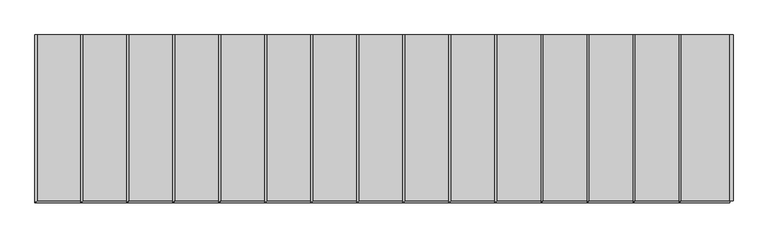
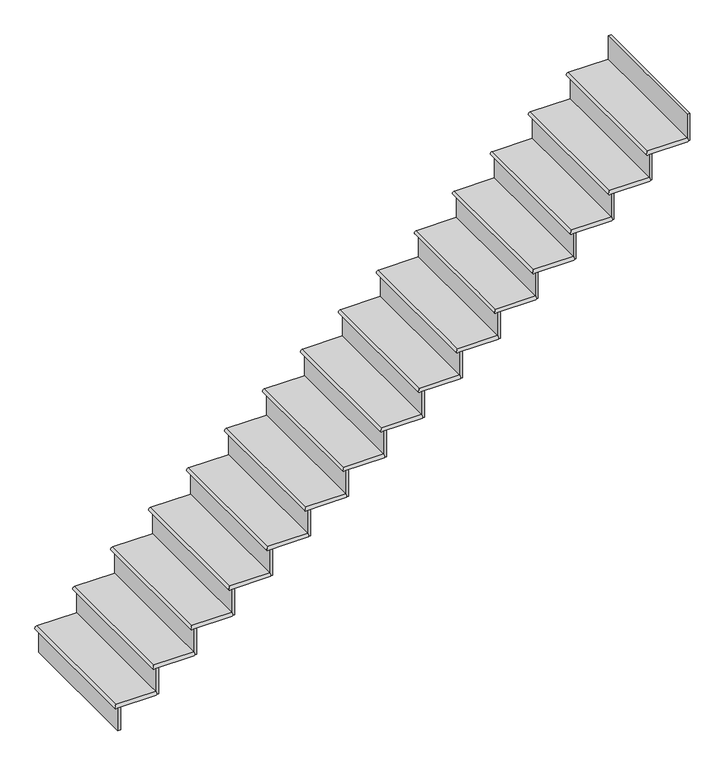
"""IFC4 building model written with IfcOpenShell, lengths in millimetres: stair flight geometry."""

import ifcopenshell
import ifcopenshell.guid

model = None  # the IFC model being written
_history = None  # IfcOwnerHistory: only IFC2X3 demands one
_inside = {}  # id of a spatial element -> (the spatial element, [elements in it])
_under = {}  # id of a project, library or spatial element -> (it, [spatial elements below it])
_declared = {}  # id of a project -> (the project, [libraries it declares])
_typed = {}  # id of a type object -> (the type object, [elements of that type])
_made_of = {}  # id of a material, layer set ... -> (it, [elements and type objects made of it])


def new_model(schema):
    """Start an empty IFC model of exactly this schema.

    Asked for "IFC4X3", IfcOpenShell would pick the latest addendum, in which some entities
    have other attributes; the version numbers below select the first issue.
    IFC2X3 requires an IfcOwnerHistory on every rooted entity: one is made here for all.
    """
    global model, _history
    if schema == "IFC4X3":
        model = ifcopenshell.file(schema_version=(4, 3, 0, 0))
    else:
        model = ifcopenshell.file(schema=schema)
    _inside.clear()
    _under.clear()
    _declared.clear()
    _typed.clear()
    _made_of.clear()
    _history = None
    if model.schema == "IFC2X3":
        org = make("IfcOrganization", Name="unknown")
        user = make(
            "IfcPersonAndOrganization",
            ThePerson=make("IfcPerson", FamilyName="unknown"),
            TheOrganization=org,
        )
        app = make(
            "IfcApplication",
            ApplicationDeveloper=org,
            Version="unknown",
            ApplicationFullName="unknown",
            ApplicationIdentifier="unknown",
        )
        _history = make(
            "IfcOwnerHistory",
            OwningUser=user,
            OwningApplication=app,
            ChangeAction="ADDED",
            CreationDate=0,
        )
    return model


def make(cls, **values):
    """One entity of the class cls with the attributes given. An attribute that is None is left unset."""
    return model.create_entity(
        cls, **{name: value for name, value in values.items() if value is not None}
    )


def rooted(cls, **values):
    """An entity with a GlobalId (a new one), such as an element, a storey or a relation."""
    return make(cls, GlobalId=ifcopenshell.guid.new(), OwnerHistory=_history, **values)


def si_unit(unit_type, name, prefix=None):
    """IfcSIUnit, for example si_unit("LENGTHUNIT", "METRE", prefix="MILLI")."""
    return make("IfcSIUnit", UnitType=unit_type, Prefix=prefix, Name=name)


def assignment(units):
    """IfcUnitAssignment: the units of a project."""
    return None if units is None else make("IfcUnitAssignment", Units=units)


def point(xyz):
    """IfcCartesianPoint."""
    return None if xyz is None else make("IfcCartesianPoint", Coordinates=xyz)


def direction(xyz):
    """IfcDirection."""
    return None if xyz is None else make("IfcDirection", DirectionRatios=xyz)


def frame(location, z_axis=None, x_axis=None):
    """IfcAxis2Placement3D, a coordinate frame: its origin and axes. An axis left out is left unset."""
    return make(
        "IfcAxis2Placement3D",
        Location=point(location),
        Axis=direction(z_axis),
        RefDirection=direction(x_axis),
    )


def origin():
    """The frame at (0, 0, 0) with its axes left unset."""
    return frame((0.0, 0.0, 0.0))


def place(relative_to, where):
    """IfcLocalPlacement: puts the frame where relative to a parent placement (None: the world)."""
    return make(
        "IfcLocalPlacement", PlacementRelTo=relative_to, RelativePlacement=where
    )


def context(
    kind, dimensions, precision=None, world=None, true_north=None, identifier=None
):
    """IfcGeometricRepresentationContext, for example the 3D "Model" context."""
    return make(
        "IfcGeometricRepresentationContext",
        ContextIdentifier=identifier,
        ContextType=kind,
        CoordinateSpaceDimension=dimensions,
        Precision=precision,
        WorldCoordinateSystem=world,
        TrueNorth=true_north,
    )


def project(units=None, contexts=None):
    """IfcProject with its units and contexts."""
    return rooted(
        "IfcProject",
        Name="project",
        RepresentationContexts=contexts,
        UnitsInContext=assignment(units),
    )


def spatial(cls, under=None, at=None, **own):
    """A site, building, storey or space (cls), placed at a placement, below another one or the project."""
    s = rooted(cls, ObjectPlacement=at, **own)
    if under is not None:
        _under.setdefault(under.id(), (under, []))[1].append(s)
    return s


def circle_curve(where, radius):
    """IfcCircle in the frame where."""
    return make("IfcCircle", Position=where, Radius=radius)


def ellipse_curve(where, semi_axis1, semi_axis2):
    """IfcEllipse in the frame where."""
    return make(
        "IfcEllipse", Position=where, SemiAxis1=semi_axis1, SemiAxis2=semi_axis2
    )


def faces_of(points, faces, orient=None, outer=None):
    """IfcFace entities. A face is a list of loops; a loop is a list of indices into points, from 0.

    orient and outer hold one flag for each loop. By default every Orientation is true, the
    first loop of a face is its IfcFaceOuterBound and the others are IfcFaceBound.
    """
    made = []
    for i, loops in enumerate(faces):
        bounds = []
        for j, loop in enumerate(loops):
            is_outer = j == 0 if outer is None else outer[i][j]
            bounds.append(
                make(
                    "IfcFaceOuterBound" if is_outer else "IfcFaceBound",
                    Bound=make("IfcPolyLoop", Polygon=[points[k] for k in loop]),
                    Orientation=True if orient is None else orient[i][j],
                )
            )
        made.append(make("IfcFace", Bounds=bounds))
    return made


def faceted_brep(points, faces, orient=None, outer=None, voids=None):
    """IfcFacetedBrep: a solid bounded by flat faces; with voids (closed shells), ...WithVoids."""
    shared = [point(p) for p in points]
    hull = make("IfcClosedShell", CfsFaces=faces_of(shared, faces, orient, outer))
    if voids is None:
        return make("IfcFacetedBrep", Outer=hull)
    return make(
        "IfcFacetedBrepWithVoids",
        Outer=hull,
        Voids=[
            make(cls, CfsFaces=faces_of(shared, fs, o, b)) for cls, fs, o, b in voids
        ],
    )


def shape(context_of_items, identifier, shape_type, items):
    """IfcShapeRepresentation: the items that make up one representation, for example the "Body"."""
    return make(
        "IfcShapeRepresentation",
        ContextOfItems=context_of_items,
        RepresentationIdentifier=identifier,
        RepresentationType=shape_type,
        Items=items,
    )


def source(mapping_origin, context_of_items, identifier, shape_type, items):
    """IfcRepresentationMap: a shape defined once, which mapped items show again and again."""
    return make(
        "IfcRepresentationMap",
        MappingOrigin=mapping_origin,
        MappedRepresentation=shape(context_of_items, identifier, shape_type, items),
    )


def transform(
    local_origin,
    x_axis=None,
    y_axis=None,
    z_axis=None,
    scale=None,
    scale2=None,
    scale3=None,
    uniform=True,
):
    """IfcCartesianTransformationOperator3D, or its non-uniform kind. x_axis, y_axis, z_axis: its Axis1, 2, 3."""
    if uniform:
        return make(
            "IfcCartesianTransformationOperator3D",
            Axis1=direction(x_axis),
            Axis2=direction(y_axis),
            LocalOrigin=point(local_origin),
            Scale=scale,
            Axis3=direction(z_axis),
        )
    return make(
        "IfcCartesianTransformationOperator3DnonUniform",
        Axis1=direction(x_axis),
        Axis2=direction(y_axis),
        LocalOrigin=point(local_origin),
        Scale=scale,
        Axis3=direction(z_axis),
        Scale2=scale2,
        Scale3=scale3,
    )


def mapped(mapping_source, mapping_target):
    """IfcMappedItem: shows the shape of a source again, moved by a transform."""
    return make(
        "IfcMappedItem", MappingSource=mapping_source, MappingTarget=mapping_target
    )


def made_of(thing, what):
    """Note that an element or type object is made of a material, layer set ...; save() writes the relation."""
    if what is not None:
        _made_of.setdefault(what.id(), (what, []))[1].append(thing)
    return thing


def element(
    cls,
    number,
    at=None,
    inside=None,
    cuts=None,
    type_object=None,
    material=None,
    context=None,
    identifier="Body",
    shape_type=None,
    held_by="IfcProductDefinitionShape",
    body=None,
    shapes=None,
    **own,
):
    """One element of the class cls, such as IfcWall. Its Tag is "e" and its number.

    at: its placement. inside: the storey or other place that contains it. cuts: it is an
    opening in that element (IfcRelVoidsElement). A single representation is given by context,
    identifier, shape_type and body (its items); several are given by shapes. held_by: the class
    of the entity that holds the representations. save() writes the other relations.
    """
    e = rooted(cls, Tag="e%d" % number, ObjectPlacement=at, **own)
    if body is not None:
        shapes = [shape(context, identifier, shape_type, body)]
    if shapes is not None:
        e.Representation = make(held_by, Representations=shapes)
    if inside is not None:
        _inside.setdefault(inside.id(), (inside, []))[1].append(e)
    if cuts is not None:
        rooted(
            "IfcRelVoidsElement", RelatingBuildingElement=cuts, RelatedOpeningElement=e
        )
    if type_object is not None:
        _typed.setdefault(type_object.id(), (type_object, []))[1].append(e)
    return made_of(e, material)


def aggregate(whole, parts):
    """IfcRelAggregates: a whole, such as a stair, and the parts it consists of."""
    return rooted("IfcRelAggregates", RelatingObject=whole, RelatedObjects=parts)


def save(model, path):
    """Write the relations noted so far, then the file.

    IfcRelAggregates (storeys below a building ...), IfcRelContainedInSpatialStructure (elements
    in a storey), IfcRelDefinesByType, IfcRelAssociatesMaterial and IfcRelDeclares: one each for
    every whole, place, type object, material and project.
    """
    for whole, parts in _under.values():
        aggregate(whole, parts)
    for where, things in _inside.values():
        rooted(
            "IfcRelContainedInSpatialStructure",
            RelatedElements=things,
            RelatingStructure=where,
        )
    for kind, things in _typed.values():
        rooted("IfcRelDefinesByType", RelatedObjects=things, RelatingType=kind)
    for what, things in _made_of.values():
        rooted("IfcRelAssociatesMaterial", RelatedObjects=things, RelatingMaterial=what)
    for by, libraries in _declared.values():
        rooted("IfcRelDeclares", RelatingContext=by, RelatedDefinitions=libraries)
    model.write(path)


def plane_surface(at):
    """IfcPlane: the flat surface through the origin of the frame at, square to its z axis."""
    return make("IfcPlane", Position=at)


def cylinder_surface(at, radius):
    """IfcCylindricalSurface: all points at the distance radius from the z axis of the frame at."""
    return make("IfcCylindricalSurface", Position=at, Radius=radius)


def advanced_brep(points, edges, surfaces, faces):
    """IfcAdvancedBrep: a solid bounded by faces that lie on surfaces and meet in shared edges.

    An edge is (start, end): straight between two places in points (the first is 0);
    or (start, end, curve); or (start, end, curve, False) where it runs against its curve.
    A face is (place in surfaces, loops), or (place, loops, False) where it looks against
    its surface's normal. A loop lists edges by number (the first is 1), with a minus sign
    where the edge is run from its end to its start. The first loop is the outer one.
    """
    corners = [point(p) for p in points]
    vertices = [make("IfcVertexPoint", VertexGeometry=c) for c in corners]
    made = []
    for start, end, *more in edges:
        made.append(
            make(
                "IfcEdgeCurve",
                EdgeStart=vertices[start],
                EdgeEnd=vertices[end],
                EdgeGeometry=more[0] if more else make("IfcPolyline", Points=[corners[start], corners[end]]),
                SameSense=more[1] if len(more) > 1 else True,
            )
        )
    hull = []
    for where, loops, *sense in faces:
        bounds = []
        for j, loop in enumerate(loops):
            ring = [make("IfcOrientedEdge", EdgeElement=made[abs(k) - 1], Orientation=k > 0) for k in loop]
            bounds.append(
                make(
                    "IfcFaceOuterBound" if j == 0 else "IfcFaceBound",
                    Bound=make("IfcEdgeLoop", EdgeList=ring),
                    Orientation=True,
                )
            )
        hull.append(make("IfcAdvancedFace", Bounds=bounds, FaceSurface=surfaces[where], SameSense=sense[0] if sense else True))
    return make("IfcAdvancedBrep", Outer=make("IfcClosedShell", CfsFaces=hull))


def stair_flight_f94ab1f9(model_context):
    return source(origin(), model_context, "Body", "SolidModel", [
        advanced_brep(
        [(-27218.1481446, 896.1568972, 165.1), (-27218.1481446, 896.1568972, 190.5), (-27218.1481446, 1810.5568972, 190.5), (-27218.1481446, 1810.5568972, 165.1), (-26951.4481446, 1810.5568972, 190.5), (-26951.4481446, 896.1568972, 190.5), (-26951.4481446, 1810.5568972, 165.1), (-26951.4481446, 896.1568972, 165.1)],
        [
            (0, 1, ellipse_curve(frame((-27218.1481446, 896.1568972, 177.8), z_axis=(-0.7071067811865447, 0.7071067811865502, 0.0), x_axis=(-0.7071067811865501, -0.7071067811865449, 0.0)), 17.9605122, 12.7)),
            (1, 2),
            (2, 3, circle_curve(frame((-27218.1481446, 1810.5568972, 177.8), z_axis=(0.0, -1.0, 0.0), x_axis=(1.0, 0.0, 0.0)), 12.7)),
            (3, 0),
            (4, 2),
            (1, 5),
            (5, 4),
            (3, 6),
            (6, 7),
            (7, 0),
            (4, 6),
            (5, 7, circle_curve(frame((-26951.4481446, 896.1568972, 177.8), z_axis=(1.0, 0.0, 0.0), x_axis=(0.0, 1.0, 0.0)), 12.7)),
        ],
        [
            cylinder_surface(frame((-27218.1481446, 896.1568972, 177.8), z_axis=(0.0, -1.0, 0.0), x_axis=(1.0, 0.0, 0.0)), 12.7),
            plane_surface(frame((-27230.8481446, 1810.5568972, 190.5), z_axis=(0.0, 0.0, 1.0), x_axis=(-1.0, 0.0, 0.0))),
            plane_surface(frame((-27230.8481446, 1810.5568972, 165.1), z_axis=(0.0, 0.0, -1.0), x_axis=(1.0, 0.0, 0.0))),
            plane_surface(frame((-26951.4481446, 1810.5568972, 190.5), z_axis=(0.0, 1.0, 0.0), x_axis=(0.0, 0.0, -1.0))),
            plane_surface(frame((-26951.4481446, 896.1568972, 190.5), z_axis=(1.0, 0.0, 0.0), x_axis=(0.0, 0.0, -1.0))),
            cylinder_surface(frame((-26951.4481446, 896.1568972, 177.8), z_axis=(1.0, 0.0, 0.0), x_axis=(0.0, 1.0, 0.0)), 12.7),
        ],
        [
            (0, [[1, 2, 3, 4]]),
            (1, [[5, -2, 6, 7]]),
            (2, [[8, 9, 10, -4]]),
            (3, [[-5, 11, -8, -3]]),
            (4, [[-7, 12, -9, -11]]),
            (5, [[-12, -6, -1, -10]]),
        ],
    ),
        faceted_brep([(-27205.4481446, 896.1568972, 165.1), (-27205.4481446, 896.1568972, 0.0), (-27186.3981446, 896.1568972, 0.0), (-27186.3981446, 896.1568972, 165.1), (-27205.4481446, 1810.5568972, 165.1), (-27186.3981446, 1810.5568972, 165.1), (-27186.3981446, 1810.5568972, 0.0), (-27205.4481446, 1810.5568972, 0.0)], [[[0, 1, 2, 3]], [[4, 5, 6, 7]], [[1, 0, 4, 7]], [[2, 1, 7, 6]], [[3, 2, 6, 5]], [[0, 3, 5, 4]]]),
        faceted_brep([(-26951.4481446, 896.1568972, 355.6), (-26951.4481446, 896.1568972, 165.1), (-26932.3981446, 896.1568972, 165.1), (-26932.3981446, 896.1568972, 355.6), (-26951.4481446, 1810.5568972, 355.6), (-26932.3981446, 1810.5568972, 355.6), (-26932.3981446, 1810.5568972, 165.1), (-26951.4481446, 1810.5568972, 165.1)], [[[0, 1, 2, 3]], [[4, 5, 6, 7]], [[1, 0, 4, 7]], [[2, 1, 7, 6]], [[3, 2, 6, 5]], [[0, 3, 5, 4]]]),
        advanced_brep(
        [(-26697.4481446, 1810.5568972, 381.0), (-26964.1481446, 1810.5568972, 381.0), (-26964.1481446, 896.1568972, 381.0), (-26697.4481446, 896.1568972, 381.0), (-26964.1481446, 1810.5568972, 355.6), (-26697.4481446, 1810.5568972, 355.6), (-26697.4481446, 896.1568972, 355.6), (-26964.1481446, 896.1568972, 355.6)],
        [
            (0, 1),
            (1, 2),
            (2, 3),
            (3, 0),
            (4, 5),
            (5, 6),
            (6, 7),
            (7, 4),
            (0, 5),
            (4, 1, circle_curve(frame((-26964.1481446, 1810.5568972, 368.3), z_axis=(0.0, 1.0, 0.0), x_axis=(1.0, 0.0, 0.0)), 12.7)),
            (3, 6, circle_curve(frame((-26697.4481446, 896.1568972, 368.3), z_axis=(1.0, 0.0, 0.0), x_axis=(0.0, 1.0, 0.0)), 12.7)),
            (7, 2, ellipse_curve(frame((-26964.1481446, 896.1568972, 368.3), z_axis=(-0.7071067811865451, 0.7071067811865499, 0.0), x_axis=(-0.7071067811865498, -0.7071067811865451, 0.0)), 17.9605122, 12.7)),
        ],
        [
            plane_surface(frame((-27230.8481446, 1810.5568972, 381.0), z_axis=(0.0, 0.0, 1.0), x_axis=(-1.0, 0.0, 0.0))),
            plane_surface(frame((-27230.8481446, 1810.5568972, 355.6), z_axis=(0.0, 0.0, -1.0), x_axis=(1.0, 0.0, 0.0))),
            plane_surface(frame((-26697.4481446, 1810.5568972, 381.0), z_axis=(0.0, 1.0, 0.0), x_axis=(0.0, 0.0, -1.0))),
            plane_surface(frame((-26697.4481446, 896.1568972, 381.0), z_axis=(1.0, 0.0, 0.0), x_axis=(0.0, 0.0, -1.0))),
            cylinder_surface(frame((-26964.1481446, 896.1568972, 368.3), z_axis=(0.0, -1.0, 0.0), x_axis=(1.0, 0.0, 0.0)), 12.7),
            cylinder_surface(frame((-26697.4481446, 896.1568972, 368.3), z_axis=(1.0, 0.0, 0.0), x_axis=(0.0, 1.0, 0.0)), 12.7),
        ],
        [
            (0, [[1, 2, 3, 4]]),
            (1, [[5, 6, 7, 8]]),
            (2, [[-1, 9, -5, 10]]),
            (3, [[-4, 11, -6, -9]]),
            (4, [[12, -2, -10, -8]]),
            (5, [[-11, -3, -12, -7]]),
        ],
    ),
        faceted_brep([(-26697.4481446, 896.1568972, 546.1), (-26697.4481446, 896.1568972, 355.6), (-26678.3981446, 896.1568972, 355.6), (-26678.3981446, 896.1568972, 546.1), (-26697.4481446, 1810.5568972, 546.1), (-26678.3981446, 1810.5568972, 546.1), (-26678.3981446, 1810.5568972, 355.6), (-26697.4481446, 1810.5568972, 355.6)], [[[0, 1, 2, 3]], [[4, 5, 6, 7]], [[1, 0, 4, 7]], [[2, 1, 7, 6]], [[3, 2, 6, 5]], [[0, 3, 5, 4]]]),
        advanced_brep(
        [(-26443.4481446, 1810.5568972, 571.5), (-26710.1481446, 1810.5568972, 571.5), (-26710.1481446, 896.1568972, 571.5), (-26443.4481446, 896.1568972, 571.5), (-26710.1481446, 1810.5568972, 546.1), (-26443.4481446, 1810.5568972, 546.1), (-26443.4481446, 896.1568972, 546.1), (-26710.1481446, 896.1568972, 546.1)],
        [
            (0, 1),
            (1, 2),
            (2, 3),
            (3, 0),
            (4, 5),
            (5, 6),
            (6, 7),
            (7, 4),
            (0, 5),
            (4, 1, circle_curve(frame((-26710.1481446, 1810.5568972, 558.8), z_axis=(0.0, 1.0, 0.0), x_axis=(1.0, 0.0, 0.0)), 12.7)),
            (3, 6, circle_curve(frame((-26443.4481446, 896.1568972, 558.8), z_axis=(1.0, 0.0, 0.0), x_axis=(0.0, 1.0, 0.0)), 12.7)),
            (7, 2, ellipse_curve(frame((-26710.1481446, 896.1568972, 558.8), z_axis=(-0.7071067811865451, 0.7071067811865499, 0.0), x_axis=(-0.7071067811865498, -0.7071067811865451, 0.0)), 17.9605122, 12.7)),
        ],
        [
            plane_surface(frame((-26976.8481446, 1810.5568972, 571.5), z_axis=(0.0, 0.0, 1.0), x_axis=(-1.0, 0.0, 0.0))),
            plane_surface(frame((-26976.8481446, 1810.5568972, 546.1), z_axis=(0.0, 0.0, -1.0), x_axis=(1.0, 0.0, 0.0))),
            plane_surface(frame((-26443.4481446, 1810.5568972, 571.5), z_axis=(0.0, 1.0, 0.0), x_axis=(0.0, 0.0, -1.0))),
            plane_surface(frame((-26443.4481446, 896.1568972, 571.5), z_axis=(1.0, 0.0, 0.0), x_axis=(0.0, 0.0, -1.0))),
            cylinder_surface(frame((-26710.1481446, 896.1568972, 558.8), z_axis=(0.0, -1.0, 0.0), x_axis=(1.0, 0.0, 0.0)), 12.7),
            cylinder_surface(frame((-26443.4481446, 896.1568972, 558.8), z_axis=(1.0, 0.0, 0.0), x_axis=(0.0, 1.0, 0.0)), 12.7),
        ],
        [
            (0, [[1, 2, 3, 4]]),
            (1, [[5, 6, 7, 8]]),
            (2, [[-1, 9, -5, 10]]),
            (3, [[-4, 11, -6, -9]]),
            (4, [[12, -2, -10, -8]]),
            (5, [[-11, -3, -12, -7]]),
        ],
    ),
        faceted_brep([(-26443.4481446, 896.1568972, 736.6), (-26443.4481446, 896.1568972, 546.1), (-26424.3981446, 896.1568972, 546.1), (-26424.3981446, 896.1568972, 736.6), (-26443.4481446, 1810.5568972, 736.6), (-26424.3981446, 1810.5568972, 736.6), (-26424.3981446, 1810.5568972, 546.1), (-26443.4481446, 1810.5568972, 546.1)], [[[0, 1, 2, 3]], [[4, 5, 6, 7]], [[1, 0, 4, 7]], [[2, 1, 7, 6]], [[3, 2, 6, 5]], [[0, 3, 5, 4]]]),
        advanced_brep(
        [(-26189.4481446, 1810.5568972, 762.0), (-26456.1481446, 1810.5568972, 762.0), (-26456.1481446, 896.1568972, 762.0), (-26189.4481446, 896.1568972, 762.0), (-26456.1481446, 1810.5568972, 736.6), (-26189.4481446, 1810.5568972, 736.6), (-26189.4481446, 896.1568972, 736.6), (-26456.1481446, 896.1568972, 736.6)],
        [
            (0, 1),
            (1, 2),
            (2, 3),
            (3, 0),
            (4, 5),
            (5, 6),
            (6, 7),
            (7, 4),
            (0, 5),
            (4, 1, circle_curve(frame((-26456.1481446, 1810.5568972, 749.3), z_axis=(0.0, 1.0, 0.0), x_axis=(1.0, 0.0, 0.0)), 12.7)),
            (3, 6, circle_curve(frame((-26189.4481446, 896.1568972, 749.3), z_axis=(1.0, 0.0, 0.0), x_axis=(0.0, 1.0, 0.0)), 12.7)),
            (7, 2, ellipse_curve(frame((-26456.1481446, 896.1568972, 749.3), z_axis=(-0.7071067811865451, 0.7071067811865499, 0.0), x_axis=(-0.7071067811865498, -0.7071067811865451, 0.0)), 17.9605122, 12.7)),
        ],
        [
            plane_surface(frame((-26722.8481446, 1810.5568972, 762.0), z_axis=(0.0, 0.0, 1.0), x_axis=(-1.0, 0.0, 0.0))),
            plane_surface(frame((-26722.8481446, 1810.5568972, 736.6), z_axis=(0.0, 0.0, -1.0), x_axis=(1.0, 0.0, 0.0))),
            plane_surface(frame((-26189.4481446, 1810.5568972, 762.0), z_axis=(0.0, 1.0, 0.0), x_axis=(0.0, 0.0, -1.0))),
            plane_surface(frame((-26189.4481446, 896.1568972, 762.0), z_axis=(1.0, 0.0, 0.0), x_axis=(0.0, 0.0, -1.0))),
            cylinder_surface(frame((-26456.1481446, 896.1568972, 749.3), z_axis=(0.0, -1.0, 0.0), x_axis=(1.0, 0.0, 0.0)), 12.7),
            cylinder_surface(frame((-26189.4481446, 896.1568972, 749.3), z_axis=(1.0, 0.0, 0.0), x_axis=(0.0, 1.0, 0.0)), 12.7),
        ],
        [
            (0, [[1, 2, 3, 4]]),
            (1, [[5, 6, 7, 8]]),
            (2, [[-1, 9, -5, 10]]),
            (3, [[-4, 11, -6, -9]]),
            (4, [[12, -2, -10, -8]]),
            (5, [[-11, -3, -12, -7]]),
        ],
    ),
        faceted_brep([(-26189.4481446, 896.1568972, 927.1), (-26189.4481446, 896.1568972, 736.6), (-26170.3981446, 896.1568972, 736.6), (-26170.3981446, 896.1568972, 927.1), (-26189.4481446, 1810.5568972, 927.1), (-26170.3981446, 1810.5568972, 927.1), (-26170.3981446, 1810.5568972, 736.6), (-26189.4481446, 1810.5568972, 736.6)], [[[0, 1, 2, 3]], [[4, 5, 6, 7]], [[1, 0, 4, 7]], [[2, 1, 7, 6]], [[3, 2, 6, 5]], [[0, 3, 5, 4]]]),
        advanced_brep(
        [(-25935.4481446, 1810.5568972, 952.5), (-26202.1481446, 1810.5568972, 952.5), (-26202.1481446, 896.1568972, 952.5), (-25935.4481446, 896.1568972, 952.5), (-26202.1481446, 1810.5568972, 927.1), (-25935.4481446, 1810.5568972, 927.1), (-25935.4481446, 896.1568972, 927.1), (-26202.1481446, 896.1568972, 927.1)],
        [
            (0, 1),
            (1, 2),
            (2, 3),
            (3, 0),
            (4, 5),
            (5, 6),
            (6, 7),
            (7, 4),
            (0, 5),
            (4, 1, circle_curve(frame((-26202.1481446, 1810.5568972, 939.8), z_axis=(0.0, 1.0, 0.0), x_axis=(1.0, 0.0, 0.0)), 12.7)),
            (3, 6, circle_curve(frame((-25935.4481446, 896.1568972, 939.8), z_axis=(1.0, 0.0, 0.0), x_axis=(0.0, 1.0, 0.0)), 12.7)),
            (7, 2, ellipse_curve(frame((-26202.1481446, 896.1568972, 939.8), z_axis=(-0.7071067811865451, 0.7071067811865499, 0.0), x_axis=(-0.7071067811865498, -0.7071067811865451, 0.0)), 17.9605122, 12.7)),
        ],
        [
            plane_surface(frame((-26468.8481446, 1810.5568972, 952.5), z_axis=(0.0, 0.0, 1.0), x_axis=(-1.0, 0.0, 0.0))),
            plane_surface(frame((-26468.8481446, 1810.5568972, 927.1), z_axis=(0.0, 0.0, -1.0), x_axis=(1.0, 0.0, 0.0))),
            plane_surface(frame((-25935.4481446, 1810.5568972, 952.5), z_axis=(0.0, 1.0, 0.0), x_axis=(0.0, 0.0, -1.0))),
            plane_surface(frame((-25935.4481446, 896.1568972, 952.5), z_axis=(1.0, 0.0, 0.0), x_axis=(0.0, 0.0, -1.0))),
            cylinder_surface(frame((-26202.1481446, 896.1568972, 939.8), z_axis=(0.0, -1.0, 0.0), x_axis=(1.0, 0.0, 0.0)), 12.7),
            cylinder_surface(frame((-25935.4481446, 896.1568972, 939.8), z_axis=(1.0, 0.0, 0.0), x_axis=(0.0, 1.0, 0.0)), 12.7),
        ],
        [
            (0, [[1, 2, 3, 4]]),
            (1, [[5, 6, 7, 8]]),
            (2, [[-1, 9, -5, 10]]),
            (3, [[-4, 11, -6, -9]]),
            (4, [[12, -2, -10, -8]]),
            (5, [[-11, -3, -12, -7]]),
        ],
    ),
        faceted_brep([(-25935.4481446, 896.1568972, 1117.6), (-25935.4481446, 896.1568972, 927.1), (-25916.3981446, 896.1568972, 927.1), (-25916.3981446, 896.1568972, 1117.6), (-25935.4481446, 1810.5568972, 1117.6), (-25916.3981446, 1810.5568972, 1117.6), (-25916.3981446, 1810.5568972, 927.1), (-25935.4481446, 1810.5568972, 927.1)], [[[0, 1, 2, 3]], [[4, 5, 6, 7]], [[1, 0, 4, 7]], [[2, 1, 7, 6]], [[3, 2, 6, 5]], [[0, 3, 5, 4]]]),
        advanced_brep(
        [(-25681.4481446, 1810.5568972, 1143.0), (-25948.1481446, 1810.5568972, 1143.0), (-25948.1481446, 896.1568972, 1143.0), (-25681.4481446, 896.1568972, 1143.0), (-25948.1481446, 1810.5568972, 1117.6), (-25681.4481446, 1810.5568972, 1117.6), (-25681.4481446, 896.1568972, 1117.6), (-25948.1481446, 896.1568972, 1117.6)],
        [
            (0, 1),
            (1, 2),
            (2, 3),
            (3, 0),
            (4, 5),
            (5, 6),
            (6, 7),
            (7, 4),
            (0, 5),
            (4, 1, circle_curve(frame((-25948.1481446, 1810.5568972, 1130.3), z_axis=(0.0, 1.0, 0.0), x_axis=(1.0, 0.0, 0.0)), 12.7)),
            (3, 6, circle_curve(frame((-25681.4481446, 896.1568972, 1130.3), z_axis=(1.0, 0.0, 0.0), x_axis=(0.0, 1.0, 0.0)), 12.7)),
            (7, 2, ellipse_curve(frame((-25948.1481446, 896.1568972, 1130.3), z_axis=(-0.7071067811865451, 0.7071067811865499, 0.0), x_axis=(-0.7071067811865498, -0.7071067811865451, 0.0)), 17.9605122, 12.7)),
        ],
        [
            plane_surface(frame((-26214.8481446, 1810.5568972, 1143.0), z_axis=(0.0, 0.0, 1.0), x_axis=(-1.0, 0.0, 0.0))),
            plane_surface(frame((-26214.8481446, 1810.5568972, 1117.6), z_axis=(0.0, 0.0, -1.0), x_axis=(1.0, 0.0, 0.0))),
            plane_surface(frame((-25681.4481446, 1810.5568972, 1143.0), z_axis=(0.0, 1.0, 0.0), x_axis=(0.0, 0.0, -1.0))),
            plane_surface(frame((-25681.4481446, 896.1568972, 1143.0), z_axis=(1.0, 0.0, 0.0), x_axis=(0.0, 0.0, -1.0))),
            cylinder_surface(frame((-25948.1481446, 896.1568972, 1130.3), z_axis=(0.0, -1.0, 0.0), x_axis=(1.0, 0.0, 0.0)), 12.7),
            cylinder_surface(frame((-25681.4481446, 896.1568972, 1130.3), z_axis=(1.0, 0.0, 0.0), x_axis=(0.0, 1.0, 0.0)), 12.7),
        ],
        [
            (0, [[1, 2, 3, 4]]),
            (1, [[5, 6, 7, 8]]),
            (2, [[-1, 9, -5, 10]]),
            (3, [[-4, 11, -6, -9]]),
            (4, [[12, -2, -10, -8]]),
            (5, [[-11, -3, -12, -7]]),
        ],
    ),
        faceted_brep([(-25681.4481446, 896.1568972, 1308.1), (-25681.4481446, 896.1568972, 1117.6), (-25662.3981446, 896.1568972, 1117.6), (-25662.3981446, 896.1568972, 1308.1), (-25681.4481446, 1810.5568972, 1308.1), (-25662.3981446, 1810.5568972, 1308.1), (-25662.3981446, 1810.5568972, 1117.6), (-25681.4481446, 1810.5568972, 1117.6)], [[[0, 1, 2, 3]], [[4, 5, 6, 7]], [[1, 0, 4, 7]], [[2, 1, 7, 6]], [[3, 2, 6, 5]], [[0, 3, 5, 4]]]),
        advanced_brep(
        [(-25427.4481446, 1810.5568972, 1333.5), (-25694.1481446, 1810.5568972, 1333.5), (-25694.1481446, 896.1568972, 1333.5), (-25427.4481446, 896.1568972, 1333.5), (-25694.1481446, 1810.5568972, 1308.1), (-25427.4481446, 1810.5568972, 1308.1), (-25427.4481446, 896.1568972, 1308.1), (-25694.1481446, 896.1568972, 1308.1)],
        [
            (0, 1),
            (1, 2),
            (2, 3),
            (3, 0),
            (4, 5),
            (5, 6),
            (6, 7),
            (7, 4),
            (0, 5),
            (4, 1, circle_curve(frame((-25694.1481446, 1810.5568972, 1320.8), z_axis=(0.0, 1.0, 0.0), x_axis=(1.0, 0.0, 0.0)), 12.7)),
            (3, 6, circle_curve(frame((-25427.4481446, 896.1568972, 1320.8), z_axis=(1.0, 0.0, 0.0), x_axis=(0.0, 1.0, 0.0)), 12.7)),
            (7, 2, ellipse_curve(frame((-25694.1481446, 896.1568972, 1320.8), z_axis=(-0.7071067811865451, 0.7071067811865499, 0.0), x_axis=(-0.7071067811865498, -0.7071067811865451, 0.0)), 17.9605122, 12.7)),
        ],
        [
            plane_surface(frame((-25960.8481446, 1810.5568972, 1333.5), z_axis=(0.0, 0.0, 1.0), x_axis=(-1.0, 0.0, 0.0))),
            plane_surface(frame((-25960.8481446, 1810.5568972, 1308.1), z_axis=(0.0, 0.0, -1.0), x_axis=(1.0, 0.0, 0.0))),
            plane_surface(frame((-25427.4481446, 1810.5568972, 1333.5), z_axis=(0.0, 1.0, 0.0), x_axis=(0.0, 0.0, -1.0))),
            plane_surface(frame((-25427.4481446, 896.1568972, 1333.5), z_axis=(1.0, 0.0, 0.0), x_axis=(0.0, 0.0, -1.0))),
            cylinder_surface(frame((-25694.1481446, 896.1568972, 1320.8), z_axis=(0.0, -1.0, 0.0), x_axis=(1.0, 0.0, 0.0)), 12.7),
            cylinder_surface(frame((-25427.4481446, 896.1568972, 1320.8), z_axis=(1.0, 0.0, 0.0), x_axis=(0.0, 1.0, 0.0)), 12.7),
        ],
        [
            (0, [[1, 2, 3, 4]]),
            (1, [[5, 6, 7, 8]]),
            (2, [[-1, 9, -5, 10]]),
            (3, [[-4, 11, -6, -9]]),
            (4, [[12, -2, -10, -8]]),
            (5, [[-11, -3, -12, -7]]),
        ],
    ),
        faceted_brep([(-25427.4481446, 896.1568972, 1498.6), (-25427.4481446, 896.1568972, 1308.1), (-25408.3981446, 896.1568972, 1308.1), (-25408.3981446, 896.1568972, 1498.6), (-25427.4481446, 1810.5568972, 1498.6), (-25408.3981446, 1810.5568972, 1498.6), (-25408.3981446, 1810.5568972, 1308.1), (-25427.4481446, 1810.5568972, 1308.1)], [[[0, 1, 2, 3]], [[4, 5, 6, 7]], [[1, 0, 4, 7]], [[2, 1, 7, 6]], [[3, 2, 6, 5]], [[0, 3, 5, 4]]]),
        advanced_brep(
        [(-25173.4481446, 1810.5568972, 1524.0), (-25440.1481446, 1810.5568972, 1524.0), (-25440.1481446, 896.1568972, 1524.0), (-25173.4481446, 896.1568972, 1524.0), (-25440.1481446, 1810.5568972, 1498.6), (-25173.4481446, 1810.5568972, 1498.6), (-25173.4481446, 896.1568972, 1498.6), (-25440.1481446, 896.1568972, 1498.6)],
        [
            (0, 1),
            (1, 2),
            (2, 3),
            (3, 0),
            (4, 5),
            (5, 6),
            (6, 7),
            (7, 4),
            (0, 5),
            (4, 1, circle_curve(frame((-25440.1481446, 1810.5568972, 1511.3), z_axis=(0.0, 1.0, 0.0), x_axis=(1.0, 0.0, 0.0)), 12.7)),
            (3, 6, circle_curve(frame((-25173.4481446, 896.1568972, 1511.3), z_axis=(1.0, 0.0, 0.0), x_axis=(0.0, 1.0, 0.0)), 12.7)),
            (7, 2, ellipse_curve(frame((-25440.1481446, 896.1568972, 1511.3), z_axis=(-0.7071067811865451, 0.7071067811865499, 0.0), x_axis=(-0.7071067811865498, -0.7071067811865451, 0.0)), 17.9605122, 12.7)),
        ],
        [
            plane_surface(frame((-25706.8481446, 1810.5568972, 1524.0), z_axis=(0.0, 0.0, 1.0), x_axis=(-1.0, 0.0, 0.0))),
            plane_surface(frame((-25706.8481446, 1810.5568972, 1498.6), z_axis=(0.0, 0.0, -1.0), x_axis=(1.0, 0.0, 0.0))),
            plane_surface(frame((-25173.4481446, 1810.5568972, 1524.0), z_axis=(0.0, 1.0, 0.0), x_axis=(0.0, 0.0, -1.0))),
            plane_surface(frame((-25173.4481446, 896.1568972, 1524.0), z_axis=(1.0, 0.0, 0.0), x_axis=(0.0, 0.0, -1.0))),
            cylinder_surface(frame((-25440.1481446, 896.1568972, 1511.3), z_axis=(0.0, -1.0, 0.0), x_axis=(1.0, 0.0, 0.0)), 12.7),
            cylinder_surface(frame((-25173.4481446, 896.1568972, 1511.3), z_axis=(1.0, 0.0, 0.0), x_axis=(0.0, 1.0, 0.0)), 12.7),
        ],
        [
            (0, [[1, 2, 3, 4]]),
            (1, [[5, 6, 7, 8]]),
            (2, [[-1, 9, -5, 10]]),
            (3, [[-4, 11, -6, -9]]),
            (4, [[12, -2, -10, -8]]),
            (5, [[-11, -3, -12, -7]]),
        ],
    ),
        faceted_brep([(-25173.4481446, 896.1568972, 1689.1), (-25173.4481446, 896.1568972, 1498.6), (-25154.3981446, 896.1568972, 1498.6), (-25154.3981446, 896.1568972, 1689.1), (-25173.4481446, 1810.5568972, 1689.1), (-25154.3981446, 1810.5568972, 1689.1), (-25154.3981446, 1810.5568972, 1498.6), (-25173.4481446, 1810.5568972, 1498.6)], [[[0, 1, 2, 3]], [[4, 5, 6, 7]], [[1, 0, 4, 7]], [[2, 1, 7, 6]], [[3, 2, 6, 5]], [[0, 3, 5, 4]]]),
        advanced_brep(
        [(-24919.4481446, 1810.5568972, 1714.5), (-25186.1481446, 1810.5568972, 1714.5), (-25186.1481446, 896.1568972, 1714.5), (-24919.4481446, 896.1568972, 1714.5), (-25186.1481446, 1810.5568972, 1689.1), (-24919.4481446, 1810.5568972, 1689.1), (-24919.4481446, 896.1568972, 1689.1), (-25186.1481446, 896.1568972, 1689.1)],
        [
            (0, 1),
            (1, 2),
            (2, 3),
            (3, 0),
            (4, 5),
            (5, 6),
            (6, 7),
            (7, 4),
            (0, 5),
            (4, 1, circle_curve(frame((-25186.1481446, 1810.5568972, 1701.8), z_axis=(0.0, 1.0, 0.0), x_axis=(1.0, 0.0, 0.0)), 12.7)),
            (3, 6, circle_curve(frame((-24919.4481446, 896.1568972, 1701.8), z_axis=(1.0, 0.0, 0.0), x_axis=(0.0, 1.0, 0.0)), 12.7)),
            (7, 2, ellipse_curve(frame((-25186.1481446, 896.1568972, 1701.8), z_axis=(-0.7071067811865451, 0.7071067811865499, 0.0), x_axis=(-0.7071067811865498, -0.7071067811865451, 0.0)), 17.9605122, 12.7)),
        ],
        [
            plane_surface(frame((-25452.8481446, 1810.5568972, 1714.5), z_axis=(0.0, 0.0, 1.0), x_axis=(-1.0, 0.0, 0.0))),
            plane_surface(frame((-25452.8481446, 1810.5568972, 1689.1), z_axis=(0.0, 0.0, -1.0), x_axis=(1.0, 0.0, 0.0))),
            plane_surface(frame((-24919.4481446, 1810.5568972, 1714.5), z_axis=(0.0, 1.0, 0.0), x_axis=(0.0, 0.0, -1.0))),
            plane_surface(frame((-24919.4481446, 896.1568972, 1714.5), z_axis=(1.0, 0.0, 0.0), x_axis=(0.0, 0.0, -1.0))),
            cylinder_surface(frame((-25186.1481446, 896.1568972, 1701.8), z_axis=(0.0, -1.0, 0.0), x_axis=(1.0, 0.0, 0.0)), 12.7),
            cylinder_surface(frame((-24919.4481446, 896.1568972, 1701.8), z_axis=(1.0, 0.0, 0.0), x_axis=(0.0, 1.0, 0.0)), 12.7),
        ],
        [
            (0, [[1, 2, 3, 4]]),
            (1, [[5, 6, 7, 8]]),
            (2, [[-1, 9, -5, 10]]),
            (3, [[-4, 11, -6, -9]]),
            (4, [[12, -2, -10, -8]]),
            (5, [[-11, -3, -12, -7]]),
        ],
    ),
        faceted_brep([(-24919.4481446, 896.1568972, 1879.6), (-24919.4481446, 896.1568972, 1689.1), (-24900.3981446, 896.1568972, 1689.1), (-24900.3981446, 896.1568972, 1879.6), (-24919.4481446, 1810.5568972, 1879.6), (-24900.3981446, 1810.5568972, 1879.6), (-24900.3981446, 1810.5568972, 1689.1), (-24919.4481446, 1810.5568972, 1689.1)], [[[0, 1, 2, 3]], [[4, 5, 6, 7]], [[1, 0, 4, 7]], [[2, 1, 7, 6]], [[3, 2, 6, 5]], [[0, 3, 5, 4]]]),
        advanced_brep(
        [(-24665.4481446, 1810.5568972, 1905.0), (-24932.1481446, 1810.5568972, 1905.0), (-24932.1481446, 896.1568972, 1905.0), (-24665.4481446, 896.1568972, 1905.0), (-24932.1481446, 1810.5568972, 1879.6), (-24665.4481446, 1810.5568972, 1879.6), (-24665.4481446, 896.1568972, 1879.6), (-24932.1481446, 896.1568972, 1879.6)],
        [
            (0, 1),
            (1, 2),
            (2, 3),
            (3, 0),
            (4, 5),
            (5, 6),
            (6, 7),
            (7, 4),
            (0, 5),
            (4, 1, circle_curve(frame((-24932.1481446, 1810.5568972, 1892.3), z_axis=(0.0, 1.0, 0.0), x_axis=(1.0, 0.0, 0.0)), 12.7)),
            (3, 6, circle_curve(frame((-24665.4481446, 896.1568972, 1892.3), z_axis=(1.0, 0.0, 0.0), x_axis=(0.0, 1.0, 0.0)), 12.7)),
            (7, 2, ellipse_curve(frame((-24932.1481446, 896.1568972, 1892.3), z_axis=(-0.7071067811865451, 0.7071067811865499, 0.0), x_axis=(-0.7071067811865498, -0.7071067811865451, 0.0)), 17.9605122, 12.7)),
        ],
        [
            plane_surface(frame((-25198.8481446, 1810.5568972, 1905.0), z_axis=(0.0, 0.0, 1.0), x_axis=(-1.0, 0.0, 0.0))),
            plane_surface(frame((-25198.8481446, 1810.5568972, 1879.6), z_axis=(0.0, 0.0, -1.0), x_axis=(1.0, 0.0, 0.0))),
            plane_surface(frame((-24665.4481446, 1810.5568972, 1905.0), z_axis=(0.0, 1.0, 0.0), x_axis=(0.0, 0.0, -1.0))),
            plane_surface(frame((-24665.4481446, 896.1568972, 1905.0), z_axis=(1.0, 0.0, 0.0), x_axis=(0.0, 0.0, -1.0))),
            cylinder_surface(frame((-24932.1481446, 896.1568972, 1892.3), z_axis=(0.0, -1.0, 0.0), x_axis=(1.0, 0.0, 0.0)), 12.7),
            cylinder_surface(frame((-24665.4481446, 896.1568972, 1892.3), z_axis=(1.0, 0.0, 0.0), x_axis=(0.0, 1.0, 0.0)), 12.7),
        ],
        [
            (0, [[1, 2, 3, 4]]),
            (1, [[5, 6, 7, 8]]),
            (2, [[-1, 9, -5, 10]]),
            (3, [[-4, 11, -6, -9]]),
            (4, [[12, -2, -10, -8]]),
            (5, [[-11, -3, -12, -7]]),
        ],
    ),
        faceted_brep([(-24665.4481446, 896.1568972, 2070.1), (-24665.4481446, 896.1568972, 1879.6), (-24646.3981446, 896.1568972, 1879.6), (-24646.3981446, 896.1568972, 2070.1), (-24665.4481446, 1810.5568972, 2070.1), (-24646.3981446, 1810.5568972, 2070.1), (-24646.3981446, 1810.5568972, 1879.6), (-24665.4481446, 1810.5568972, 1879.6)], [[[0, 1, 2, 3]], [[4, 5, 6, 7]], [[1, 0, 4, 7]], [[2, 1, 7, 6]], [[3, 2, 6, 5]], [[0, 3, 5, 4]]]),
        advanced_brep(
        [(-24411.4481446, 1810.5568972, 2095.5), (-24678.1481446, 1810.5568972, 2095.5), (-24678.1481446, 896.1568972, 2095.5), (-24411.4481446, 896.1568972, 2095.5), (-24678.1481446, 1810.5568972, 2070.1), (-24411.4481446, 1810.5568972, 2070.1), (-24411.4481446, 896.1568972, 2070.1), (-24678.1481446, 896.1568972, 2070.1)],
        [
            (0, 1),
            (1, 2),
            (2, 3),
            (3, 0),
            (4, 5),
            (5, 6),
            (6, 7),
            (7, 4),
            (0, 5),
            (4, 1, circle_curve(frame((-24678.1481446, 1810.5568972, 2082.8), z_axis=(0.0, 1.0, 0.0), x_axis=(1.0, 0.0, 0.0)), 12.7)),
            (3, 6, circle_curve(frame((-24411.4481446, 896.1568972, 2082.8), z_axis=(1.0, 0.0, 0.0), x_axis=(0.0, 1.0, 0.0)), 12.7)),
            (7, 2, ellipse_curve(frame((-24678.1481446, 896.1568972, 2082.8), z_axis=(-0.7071067811865451, 0.7071067811865499, 0.0), x_axis=(-0.7071067811865498, -0.7071067811865451, 0.0)), 17.9605122, 12.7)),
        ],
        [
            plane_surface(frame((-24944.8481446, 1810.5568972, 2095.5), z_axis=(0.0, 0.0, 1.0), x_axis=(-1.0, 0.0, 0.0))),
            plane_surface(frame((-24944.8481446, 1810.5568972, 2070.1), z_axis=(0.0, 0.0, -1.0), x_axis=(1.0, 0.0, 0.0))),
            plane_surface(frame((-24411.4481446, 1810.5568972, 2095.5), z_axis=(0.0, 1.0, 0.0), x_axis=(0.0, 0.0, -1.0))),
            plane_surface(frame((-24411.4481446, 896.1568972, 2095.5), z_axis=(1.0, 0.0, 0.0), x_axis=(0.0, 0.0, -1.0))),
            cylinder_surface(frame((-24678.1481446, 896.1568972, 2082.8), z_axis=(0.0, -1.0, 0.0), x_axis=(1.0, 0.0, 0.0)), 12.7),
            cylinder_surface(frame((-24411.4481446, 896.1568972, 2082.8), z_axis=(1.0, 0.0, 0.0), x_axis=(0.0, 1.0, 0.0)), 12.7),
        ],
        [
            (0, [[1, 2, 3, 4]]),
            (1, [[5, 6, 7, 8]]),
            (2, [[-1, 9, -5, 10]]),
            (3, [[-4, 11, -6, -9]]),
            (4, [[12, -2, -10, -8]]),
            (5, [[-11, -3, -12, -7]]),
        ],
    ),
        faceted_brep([(-24411.4481446, 896.1568972, 2260.6), (-24411.4481446, 896.1568972, 2070.1), (-24392.3981446, 896.1568972, 2070.1), (-24392.3981446, 896.1568972, 2260.6), (-24411.4481446, 1810.5568972, 2260.6), (-24392.3981446, 1810.5568972, 2260.6), (-24392.3981446, 1810.5568972, 2070.1), (-24411.4481446, 1810.5568972, 2070.1)], [[[0, 1, 2, 3]], [[4, 5, 6, 7]], [[1, 0, 4, 7]], [[2, 1, 7, 6]], [[3, 2, 6, 5]], [[0, 3, 5, 4]]]),
        advanced_brep(
        [(-24157.4481446, 1810.5568972, 2286.0), (-24424.1481446, 1810.5568972, 2286.0), (-24424.1481446, 896.1568972, 2286.0), (-24157.4481446, 896.1568972, 2286.0), (-24424.1481446, 1810.5568972, 2260.6), (-24157.4481446, 1810.5568972, 2260.6), (-24157.4481446, 896.1568972, 2260.6), (-24424.1481446, 896.1568972, 2260.6)],
        [
            (0, 1),
            (1, 2),
            (2, 3),
            (3, 0),
            (4, 5),
            (5, 6),
            (6, 7),
            (7, 4),
            (0, 5),
            (4, 1, circle_curve(frame((-24424.1481446, 1810.5568972, 2273.3), z_axis=(0.0, 1.0, 0.0), x_axis=(1.0, 0.0, 0.0)), 12.7)),
            (3, 6, circle_curve(frame((-24157.4481446, 896.1568972, 2273.3), z_axis=(1.0, 0.0, 0.0), x_axis=(0.0, 1.0, 0.0)), 12.7)),
            (7, 2, ellipse_curve(frame((-24424.1481446, 896.1568972, 2273.3), z_axis=(-0.7071067811865451, 0.7071067811865499, 0.0), x_axis=(-0.7071067811865498, -0.7071067811865451, 0.0)), 17.9605122, 12.7)),
        ],
        [
            plane_surface(frame((-24690.8481446, 1810.5568972, 2286.0), z_axis=(0.0, 0.0, 1.0), x_axis=(-1.0, 0.0, 0.0))),
            plane_surface(frame((-24690.8481446, 1810.5568972, 2260.6), z_axis=(0.0, 0.0, -1.0), x_axis=(1.0, 0.0, 0.0))),
            plane_surface(frame((-24157.4481446, 1810.5568972, 2286.0), z_axis=(0.0, 1.0, 0.0), x_axis=(0.0, 0.0, -1.0))),
            plane_surface(frame((-24157.4481446, 896.1568972, 2286.0), z_axis=(1.0, 0.0, 0.0), x_axis=(0.0, 0.0, -1.0))),
            cylinder_surface(frame((-24424.1481446, 896.1568972, 2273.3), z_axis=(0.0, -1.0, 0.0), x_axis=(1.0, 0.0, 0.0)), 12.7),
            cylinder_surface(frame((-24157.4481446, 896.1568972, 2273.3), z_axis=(1.0, 0.0, 0.0), x_axis=(0.0, 1.0, 0.0)), 12.7),
        ],
        [
            (0, [[1, 2, 3, 4]]),
            (1, [[5, 6, 7, 8]]),
            (2, [[-1, 9, -5, 10]]),
            (3, [[-4, 11, -6, -9]]),
            (4, [[12, -2, -10, -8]]),
            (5, [[-11, -3, -12, -7]]),
        ],
    ),
        faceted_brep([(-24157.4481446, 896.1568972, 2451.1), (-24157.4481446, 896.1568972, 2260.6), (-24138.3981446, 896.1568972, 2260.6), (-24138.3981446, 896.1568972, 2451.1), (-24157.4481446, 1810.5568972, 2451.1), (-24138.3981446, 1810.5568972, 2451.1), (-24138.3981446, 1810.5568972, 2260.6), (-24157.4481446, 1810.5568972, 2260.6)], [[[0, 1, 2, 3]], [[4, 5, 6, 7]], [[1, 0, 4, 7]], [[2, 1, 7, 6]], [[3, 2, 6, 5]], [[0, 3, 5, 4]]]),
        advanced_brep(
        [(-23903.4481446, 1810.5568972, 2476.5), (-24170.1481446, 1810.5568972, 2476.5), (-24170.1481446, 896.1568972, 2476.5), (-23903.4481446, 896.1568972, 2476.5), (-24170.1481446, 1810.5568972, 2451.1), (-23903.4481446, 1810.5568972, 2451.1), (-23903.4481446, 896.1568972, 2451.1), (-24170.1481446, 896.1568972, 2451.1)],
        [
            (0, 1),
            (1, 2),
            (2, 3),
            (3, 0),
            (4, 5),
            (5, 6),
            (6, 7),
            (7, 4),
            (0, 5),
            (4, 1, circle_curve(frame((-24170.1481446, 1810.5568972, 2463.8), z_axis=(0.0, 1.0, 0.0), x_axis=(1.0, 0.0, 0.0)), 12.7)),
            (3, 6, circle_curve(frame((-23903.4481446, 896.1568972, 2463.8), z_axis=(1.0, 0.0, 0.0), x_axis=(0.0, 1.0, 0.0)), 12.7)),
            (7, 2, ellipse_curve(frame((-24170.1481446, 896.1568972, 2463.8), z_axis=(-0.7071067811865451, 0.7071067811865499, 0.0), x_axis=(-0.7071067811865498, -0.7071067811865451, 0.0)), 17.9605122, 12.7)),
        ],
        [
            plane_surface(frame((-24436.8481446, 1810.5568972, 2476.5), z_axis=(0.0, 0.0, 1.0), x_axis=(-1.0, 0.0, 0.0))),
            plane_surface(frame((-24436.8481446, 1810.5568972, 2451.1), z_axis=(0.0, 0.0, -1.0), x_axis=(1.0, 0.0, 0.0))),
            plane_surface(frame((-23903.4481446, 1810.5568972, 2476.5), z_axis=(0.0, 1.0, 0.0), x_axis=(0.0, 0.0, -1.0))),
            plane_surface(frame((-23903.4481446, 896.1568972, 2476.5), z_axis=(1.0, 0.0, 0.0), x_axis=(0.0, 0.0, -1.0))),
            cylinder_surface(frame((-24170.1481446, 896.1568972, 2463.8), z_axis=(0.0, -1.0, 0.0), x_axis=(1.0, 0.0, 0.0)), 12.7),
            cylinder_surface(frame((-23903.4481446, 896.1568972, 2463.8), z_axis=(1.0, 0.0, 0.0), x_axis=(0.0, 1.0, 0.0)), 12.7),
        ],
        [
            (0, [[1, 2, 3, 4]]),
            (1, [[5, 6, 7, 8]]),
            (2, [[-1, 9, -5, 10]]),
            (3, [[-4, 11, -6, -9]]),
            (4, [[12, -2, -10, -8]]),
            (5, [[-11, -3, -12, -7]]),
        ],
    ),
        faceted_brep([(-23903.4481446, 896.1568972, 2641.6), (-23903.4481446, 896.1568972, 2451.1), (-23884.3981446, 896.1568972, 2451.1), (-23884.3981446, 896.1568972, 2641.6), (-23903.4481446, 1810.5568972, 2641.6), (-23884.3981446, 1810.5568972, 2641.6), (-23884.3981446, 1810.5568972, 2451.1), (-23903.4481446, 1810.5568972, 2451.1)], [[[0, 1, 2, 3]], [[4, 5, 6, 7]], [[1, 0, 4, 7]], [[2, 1, 7, 6]], [[3, 2, 6, 5]], [[0, 3, 5, 4]]]),
        advanced_brep(
        [(-23649.4481446, 1810.5568972, 2667.0), (-23916.1481446, 1810.5568972, 2667.0), (-23916.1481446, 896.1568972, 2667.0), (-23649.4481446, 896.1568972, 2667.0), (-23916.1481446, 1810.5568972, 2641.6), (-23649.4481446, 1810.5568972, 2641.6), (-23649.4481446, 896.1568972, 2641.6), (-23916.1481446, 896.1568972, 2641.6)],
        [
            (0, 1),
            (1, 2),
            (2, 3),
            (3, 0),
            (4, 5),
            (5, 6),
            (6, 7),
            (7, 4),
            (0, 5),
            (4, 1, circle_curve(frame((-23916.1481446, 1810.5568972, 2654.3), z_axis=(0.0, 1.0, 0.0), x_axis=(1.0, 0.0, 0.0)), 12.7)),
            (3, 6, circle_curve(frame((-23649.4481446, 896.1568972, 2654.3), z_axis=(1.0, 0.0, 0.0), x_axis=(0.0, 1.0, 0.0)), 12.7)),
            (7, 2, ellipse_curve(frame((-23916.1481446, 896.1568972, 2654.3), z_axis=(-0.7071067811865451, 0.7071067811865499, 0.0), x_axis=(-0.7071067811865498, -0.7071067811865451, 0.0)), 17.9605122, 12.7)),
        ],
        [
            plane_surface(frame((-24182.8481446, 1810.5568972, 2667.0), z_axis=(0.0, 0.0, 1.0), x_axis=(-1.0, 0.0, 0.0))),
            plane_surface(frame((-24182.8481446, 1810.5568972, 2641.6), z_axis=(0.0, 0.0, -1.0), x_axis=(1.0, 0.0, 0.0))),
            plane_surface(frame((-23649.4481446, 1810.5568972, 2667.0), z_axis=(0.0, 1.0, 0.0), x_axis=(0.0, 0.0, -1.0))),
            plane_surface(frame((-23649.4481446, 896.1568972, 2667.0), z_axis=(1.0, 0.0, 0.0), x_axis=(0.0, 0.0, -1.0))),
            cylinder_surface(frame((-23916.1481446, 896.1568972, 2654.3), z_axis=(0.0, -1.0, 0.0), x_axis=(1.0, 0.0, 0.0)), 12.7),
            cylinder_surface(frame((-23649.4481446, 896.1568972, 2654.3), z_axis=(1.0, 0.0, 0.0), x_axis=(0.0, 1.0, 0.0)), 12.7),
        ],
        [
            (0, [[1, 2, 3, 4]]),
            (1, [[5, 6, 7, 8]]),
            (2, [[-1, 9, -5, 10]]),
            (3, [[-4, 11, -6, -9]]),
            (4, [[12, -2, -10, -8]]),
            (5, [[-11, -3, -12, -7]]),
        ],
    ),
        faceted_brep([(-23649.4481446, 896.1568972, 2832.1), (-23649.4481446, 896.1568972, 2641.6), (-23630.3981446, 896.1568972, 2641.6), (-23630.3981446, 896.1568972, 2832.1), (-23649.4481446, 1810.5568972, 2832.1), (-23630.3981446, 1810.5568972, 2832.1), (-23630.3981446, 1810.5568972, 2641.6), (-23649.4481446, 1810.5568972, 2641.6)], [[[0, 1, 2, 3]], [[4, 5, 6, 7]], [[1, 0, 4, 7]], [[2, 1, 7, 6]], [[3, 2, 6, 5]], [[0, 3, 5, 4]]]),
        faceted_brep([(-23395.4481446, 896.1568972, 3022.6), (-23395.4481446, 896.1568972, 2832.1), (-23376.3981446, 896.1568972, 2832.1), (-23376.3981446, 896.1568972, 3022.6), (-23395.4481446, 1810.5568972, 3022.6), (-23376.3981446, 1810.5568972, 3022.6), (-23376.3981446, 1810.5568972, 2832.1), (-23395.4481446, 1810.5568972, 2832.1)], [[[0, 1, 2, 3]], [[4, 5, 6, 7]], [[1, 0, 4, 7]], [[2, 1, 7, 6]], [[3, 2, 6, 5]], [[0, 3, 5, 4]]]),
        advanced_brep(
        [(-23395.4481446, 1810.5568972, 2857.5), (-23662.1481446, 1810.5568972, 2857.5), (-23662.1481446, 896.1568972, 2857.5), (-23395.4481446, 896.1568972, 2857.5), (-23662.1481446, 1810.5568972, 2832.1), (-23395.4481446, 1810.5568972, 2832.1), (-23395.4481446, 896.1568972, 2832.1), (-23662.1481446, 896.1568972, 2832.1)],
        [
            (0, 1),
            (1, 2),
            (2, 3),
            (3, 0),
            (4, 5),
            (5, 6),
            (6, 7),
            (7, 4),
            (0, 5),
            (4, 1, circle_curve(frame((-23662.1481446, 1810.5568972, 2844.8), z_axis=(0.0, 1.0, 0.0), x_axis=(1.0, 0.0, 0.0)), 12.7)),
            (3, 6, circle_curve(frame((-23395.4481446, 896.1568972, 2844.8), z_axis=(1.0, 0.0, 0.0), x_axis=(0.0, 1.0, 0.0)), 12.7)),
            (7, 2, ellipse_curve(frame((-23662.1481446, 896.1568972, 2844.8), z_axis=(-0.7071067811865451, 0.7071067811865499, 0.0), x_axis=(-0.7071067811865498, -0.7071067811865451, 0.0)), 17.9605122, 12.7)),
        ],
        [
            plane_surface(frame((-23928.8481446, 1810.5568972, 2857.5), z_axis=(0.0, 0.0, 1.0), x_axis=(-1.0, 0.0, 0.0))),
            plane_surface(frame((-23928.8481446, 1810.5568972, 2832.1), z_axis=(0.0, 0.0, -1.0), x_axis=(1.0, 0.0, 0.0))),
            plane_surface(frame((-23395.4481446, 1810.5568972, 2857.5), z_axis=(0.0, 1.0, 0.0), x_axis=(0.0, 0.0, -1.0))),
            plane_surface(frame((-23395.4481446, 896.1568972, 2857.5), z_axis=(1.0, 0.0, 0.0), x_axis=(0.0, 0.0, -1.0))),
            cylinder_surface(frame((-23662.1481446, 896.1568972, 2844.8), z_axis=(0.0, -1.0, 0.0), x_axis=(1.0, 0.0, 0.0)), 12.7),
            cylinder_surface(frame((-23395.4481446, 896.1568972, 2844.8), z_axis=(1.0, 0.0, 0.0), x_axis=(0.0, 1.0, 0.0)), 12.7),
        ],
        [
            (0, [[1, 2, 3, 4]]),
            (1, [[5, 6, 7, 8]]),
            (2, [[-1, 9, -5, 10]]),
            (3, [[-4, 11, -6, -9]]),
            (4, [[12, -2, -10, -8]]),
            (5, [[-11, -3, -12, -7]]),
        ],
    ),
    ])


if __name__ == "__main__":
    model = new_model("IFC4")
    model_context = context("Model", 3, world=origin())
    ifc_project = project(units=[si_unit("LENGTHUNIT", "METRE", prefix="MILLI")], contexts=[model_context])
    site = spatial("IfcSite", under=ifc_project)
    building = spatial("IfcBuilding", under=site)
    placement = place(None, origin())
    stair_flight_shape = stair_flight_f94ab1f9(model_context)
    element("IfcStairFlight", 1, at=placement, inside=building, context=model_context, shape_type="MappedRepresentation", body=[
        mapped(stair_flight_shape, transform((0.0, 0.0, 0.0), x_axis=(1.0, 0.0, 0.0), y_axis=(0.0, 1.0, 0.0), z_axis=(0.0, 0.0, 1.0))),
    ])
    save(model, "model.ifc")

# Revit data of these elements
# Element 1 (IfcStairFlight)
#   Materials on its faces: "Wood - Cherry"
# Materials
#   "Wood - Cherry": class "Unassigned", colour RGB 226 177 128, transparency 0
